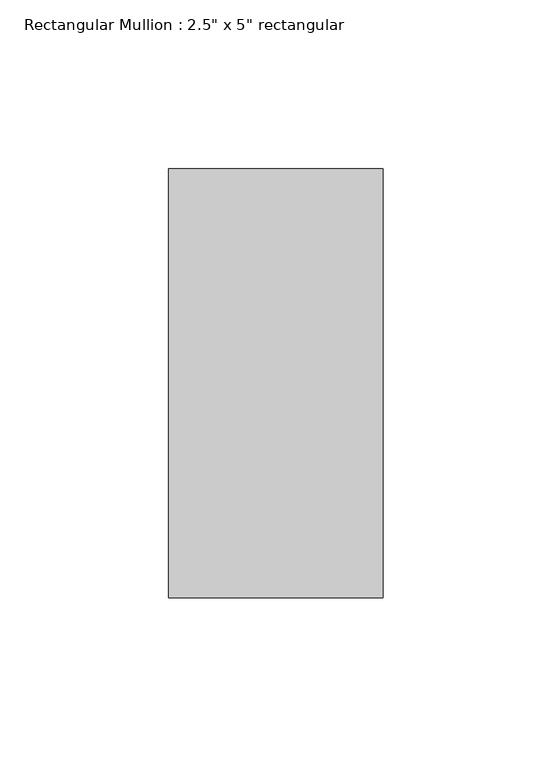
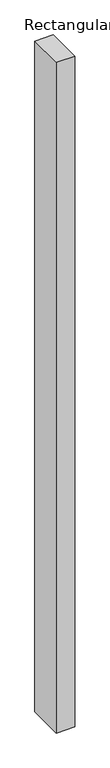
"""IFC4 building model written with IfcOpenShell, lengths in millimetres: member geometry."""

from ifc_helpers import new_model, si_unit, frame, origin, place, context, project, spatial, polyline, outline, extrude, source, transform, mapped, element, save


def member_ee409385(model_context):
    return source(origin(), model_context, "Body", "SweptSolid", [
        extrude(outline(polyline([(0.0, 63.5), (0.0, -63.5), (-63.5, -63.5), (-63.5, 63.5), (0.0, 63.5)])), frame((0.0, 0.0, -2438.4), z_axis=(0.0, 0.0, 1.0), x_axis=(1.0, 0.0, 0.0)), (0.0, 0.0, 1.0), 2438.4),
    ])


if __name__ == "__main__":
    model = new_model("IFC4")
    model_context = context("Model", 3, world=origin())
    ifc_project = project(units=[si_unit("LENGTHUNIT", "METRE", prefix="MILLI")], contexts=[model_context])
    site = spatial("IfcSite", under=ifc_project)
    building = spatial("IfcBuilding", under=site)
    placement = place(None, origin())
    member_shape = member_ee409385(model_context)
    element("IfcMember", 1, ObjectType="Rectangular Mullion : 2.5\" x 5\" rectangular", at=placement, inside=building, context=model_context, shape_type="MappedRepresentation", body=[
        mapped(member_shape, transform((0.0, 0.0, 0.0), x_axis=(1.0, 0.0, 0.0), y_axis=(0.0, 1.0, 0.0), z_axis=(0.0, 0.0, 1.0))),
    ])
    save(model, "model.ifc")

# Revit data of these elements
# Type "Rectangular Mullion : 2.5\" x 5\" rectangular"
#   built-in parameter 1007304 = 0.416667 (stored number, unit not read)
#   built-in parameter 1007301 = 0.104167 (stored number, unit not read)
#   built-in parameter 1007300 = 0.104167 (stored number, unit not read)
# Element 1 (IfcMember, "Rectangular Mullion : 2.5\" x 5\" rectangular")
#   Materials on its faces: "Metal - Aluminum"
# Materials
#   "Metal - Aluminum": class "Metal", colour RGB 140 140 140, transparency 0
